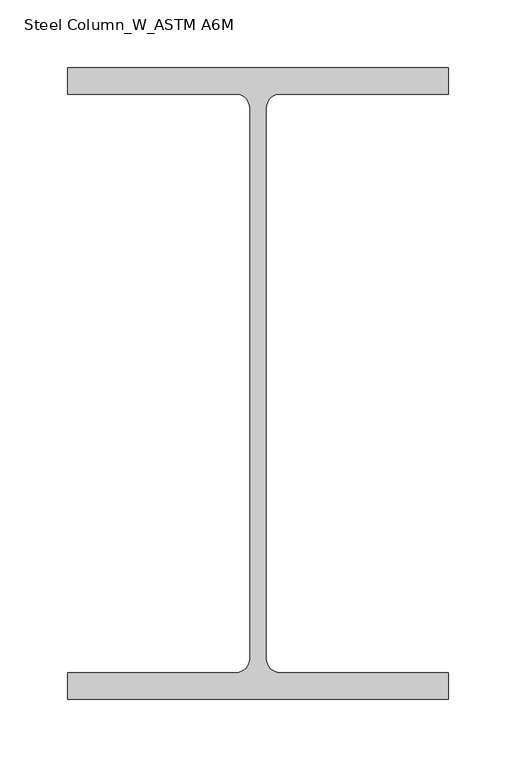
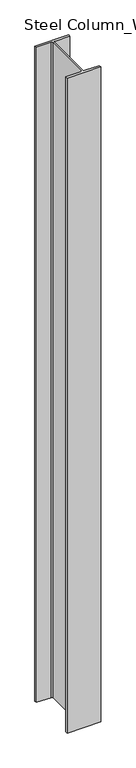
"""IFC4 building model written with IfcOpenShell, lengths in millimetres: column geometry, Steel Column_W_ASTM A6M : H_SC_AR_S01_W460x128_C1."""

from ifc_helpers import new_model, si_unit, point, frame, frame_2d, origin, place, context, project, spatial, polyline, circle_curve, trimmed, segment, composite_curve, outline, extrude, source, transform, mapped, element, save


def steel_column_w_astm_a6m_ab34c4d8(model_context):
    return source(origin(), model_context, "Body", "SweptSolid", [
        extrude(outline(composite_curve([segment(polyline([(141.0, 233.5), (141.0, 213.9), (16.2, 213.9)]), True, "CONTINUOUS"), segment(trimmed(circle_curve(frame_2d((16.2, 203.8)), 10.1), [point((16.2, 213.9))], [point((6.1, 203.8))], True, "CARTESIAN"), True, "CONTINUOUS"), segment(polyline([(6.1, 203.8), (6.1, -203.8)]), True, "CONTINUOUS"), segment(trimmed(circle_curve(frame_2d((16.2, -203.8)), 10.1), [point((6.1, -203.8))], [point((16.2, -213.9))], True, "CARTESIAN"), True, "CONTINUOUS"), segment(polyline([(16.2, -213.9), (141.0, -213.9), (141.0, -233.5), (-141.0, -233.5), (-141.0, -213.9), (-16.2, -213.9)]), True, "CONTINUOUS"), segment(trimmed(circle_curve(frame_2d((-16.2, -203.8)), 10.1), [point((-16.2, -213.9))], [point((-6.1, -203.8))], True, "CARTESIAN"), True, "CONTINUOUS"), segment(polyline([(-6.1, -203.8), (-6.1, 203.8)]), True, "CONTINUOUS"), segment(trimmed(circle_curve(frame_2d((-16.2, 203.8)), 10.1), [point((-6.1, 203.8))], [point((-16.2, 213.9))], True, "CARTESIAN"), True, "CONTINUOUS"), segment(polyline([(-16.2, 213.9), (-141.0, 213.9), (-141.0, 233.5), (141.0, 233.5)]), True, "CONTINUOUS")], self_intersect=False)), frame((0.0, 0.0, 3519.8243501), z_axis=(0.0, 0.0, 1.0), x_axis=(1.0, 0.0, 0.0)), (0.0, 0.0, 1.0), 5800.0),
    ])


if __name__ == "__main__":
    model = new_model("IFC4")
    model_context = context("Model", 3, world=origin())
    ifc_project = project(units=[si_unit("LENGTHUNIT", "METRE", prefix="MILLI")], contexts=[model_context])
    site = spatial("IfcSite", under=ifc_project)
    building = spatial("IfcBuilding", under=site)
    placement = place(None, origin())
    steel_column_w_astm_a6m_shape = steel_column_w_astm_a6m_ab34c4d8(model_context)
    element("IfcColumn", 1, ObjectType="Steel Column_W_ASTM A6M : H_SC_AR_S01_W460x128_C1", at=placement, inside=building, context=model_context, shape_type="MappedRepresentation", body=[
        mapped(steel_column_w_astm_a6m_shape, transform((0.0, 0.0, 0.0), x_axis=(1.0, 0.0, 0.0), y_axis=(0.0, 1.0, 0.0), z_axis=(0.0, 0.0, 1.0))),
    ])
    save(model, "model.ifc")

# Revit data of these elements
# Type "Steel Column_W_ASTM A6M : H_SC_AR_S01_W460x128_C1"
#   Section Name Key = "W18x86"
#   Width = 28.2 cm
#   Web Thickness = 1.22 cm
#   Web Fillet = 1.01 cm
#   Warping Constant = 3650000.0 cm⁶
#   Torsional Moment of Inertia = 171.00 cm⁴
#   Section Area = 163.0 cm²
#   Plastic Modulus weak axis = 793.0 cm³
#   Plastic Modulus strong axis = 3050.0 cm³
#   Perimeter = 2.02 m²/m
#   Nominal Weight = 128.00 kgf/m
#   Moment of Inertia weak axis = 7280.00 cm⁴
#   Moment of Inertia strong axis = 63700.00 cm⁴
#   Height = 46.7 cm
#   Flange Thickness = 1.96 cm
#   Elastic Modulus weak axis = 518.0 cm³
#   Elastic Modulus strong axis = 2720.0 cm³
#   Centroid Vertical = 23.35 cm
#   Centroid Horizontal = 14.1 cm
#   Structural Material [instance default] = Steel, 45-345
#   Bolt Spacing = 0
#   Assembly Code = ""
# Element 1 (IfcColumn, "Steel Column_W_ASTM A6M : H_SC_AR_S01_W460x128_C1")
#   Structural Material = Steel ASTM A992 GRADE 50
#   Materials on its faces: "Steel ASTM A992 GRADE 50"
# Materials
#   "Steel, 45-345": class "Metal", colour RGB 189 187 185, transparency 0, Description = "Steel 345 MPa", Cost = 0
#   "Steel ASTM A992 GRADE 50": class "Metal", colour RGB 120 120 120, transparency 0, Description = "Structural steel 50ksi", Cost = 0
